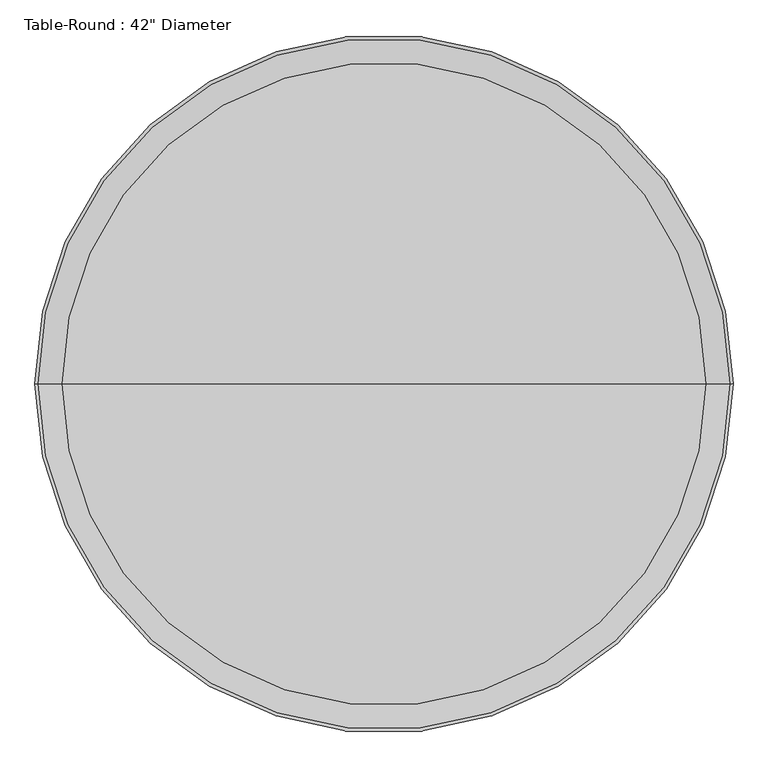
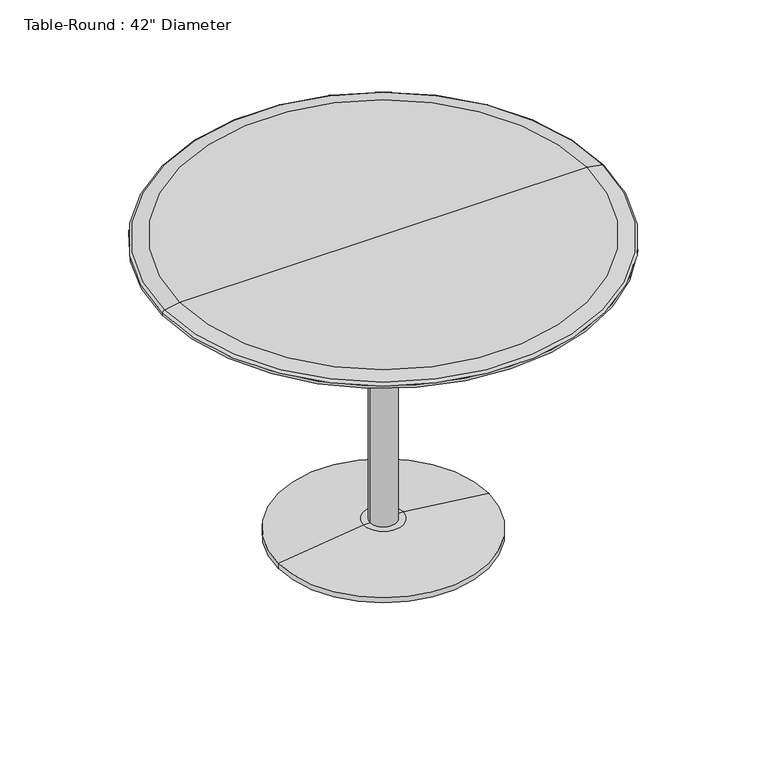
"""IFC4 building model written with IfcOpenShell, lengths in millimetres: furniture geometry."""

import ifcopenshell
import ifcopenshell.guid

model = None  # the IFC model being written
_history = None  # IfcOwnerHistory: only IFC2X3 demands one
_inside = {}  # id of a spatial element -> (the spatial element, [elements in it])
_under = {}  # id of a project, library or spatial element -> (it, [spatial elements below it])
_declared = {}  # id of a project -> (the project, [libraries it declares])
_typed = {}  # id of a type object -> (the type object, [elements of that type])
_made_of = {}  # id of a material, layer set ... -> (it, [elements and type objects made of it])


def new_model(schema):
    """Start an empty IFC model of exactly this schema.

    Asked for "IFC4X3", IfcOpenShell would pick the latest addendum, in which some entities
    have other attributes; the version numbers below select the first issue.
    IFC2X3 requires an IfcOwnerHistory on every rooted entity: one is made here for all.
    """
    global model, _history
    if schema == "IFC4X3":
        model = ifcopenshell.file(schema_version=(4, 3, 0, 0))
    else:
        model = ifcopenshell.file(schema=schema)
    _inside.clear()
    _under.clear()
    _declared.clear()
    _typed.clear()
    _made_of.clear()
    _history = None
    if model.schema == "IFC2X3":
        org = make("IfcOrganization", Name="unknown")
        user = make(
            "IfcPersonAndOrganization",
            ThePerson=make("IfcPerson", FamilyName="unknown"),
            TheOrganization=org,
        )
        app = make(
            "IfcApplication",
            ApplicationDeveloper=org,
            Version="unknown",
            ApplicationFullName="unknown",
            ApplicationIdentifier="unknown",
        )
        _history = make(
            "IfcOwnerHistory",
            OwningUser=user,
            OwningApplication=app,
            ChangeAction="ADDED",
            CreationDate=0,
        )
    return model


def make(cls, **values):
    """One entity of the class cls with the attributes given. An attribute that is None is left unset."""
    return model.create_entity(
        cls, **{name: value for name, value in values.items() if value is not None}
    )


def rooted(cls, **values):
    """An entity with a GlobalId (a new one), such as an element, a storey or a relation."""
    return make(cls, GlobalId=ifcopenshell.guid.new(), OwnerHistory=_history, **values)


def si_unit(unit_type, name, prefix=None):
    """IfcSIUnit, for example si_unit("LENGTHUNIT", "METRE", prefix="MILLI")."""
    return make("IfcSIUnit", UnitType=unit_type, Prefix=prefix, Name=name)


def assignment(units):
    """IfcUnitAssignment: the units of a project."""
    return None if units is None else make("IfcUnitAssignment", Units=units)


def point(xyz):
    """IfcCartesianPoint."""
    return None if xyz is None else make("IfcCartesianPoint", Coordinates=xyz)


def direction(xyz):
    """IfcDirection."""
    return None if xyz is None else make("IfcDirection", DirectionRatios=xyz)


def frame(location, z_axis=None, x_axis=None):
    """IfcAxis2Placement3D, a coordinate frame: its origin and axes. An axis left out is left unset."""
    return make(
        "IfcAxis2Placement3D",
        Location=point(location),
        Axis=direction(z_axis),
        RefDirection=direction(x_axis),
    )


def frame_2d(location, x_axis=None):
    """IfcAxis2Placement2D, a coordinate frame in the plane: its origin and x axis."""
    return make(
        "IfcAxis2Placement2D", Location=point(location), RefDirection=direction(x_axis)
    )


def origin():
    """The frame at (0, 0, 0) with its axes left unset."""
    return frame((0.0, 0.0, 0.0))


def origin_2d():
    """The frame at (0, 0) in the plane with its x axis left unset."""
    return frame_2d((0.0, 0.0))


def place(relative_to, where):
    """IfcLocalPlacement: puts the frame where relative to a parent placement (None: the world)."""
    return make(
        "IfcLocalPlacement", PlacementRelTo=relative_to, RelativePlacement=where
    )


def context(
    kind, dimensions, precision=None, world=None, true_north=None, identifier=None
):
    """IfcGeometricRepresentationContext, for example the 3D "Model" context."""
    return make(
        "IfcGeometricRepresentationContext",
        ContextIdentifier=identifier,
        ContextType=kind,
        CoordinateSpaceDimension=dimensions,
        Precision=precision,
        WorldCoordinateSystem=world,
        TrueNorth=true_north,
    )


def project(units=None, contexts=None):
    """IfcProject with its units and contexts."""
    return rooted(
        "IfcProject",
        Name="project",
        RepresentationContexts=contexts,
        UnitsInContext=assignment(units),
    )


def spatial(cls, under=None, at=None, **own):
    """A site, building, storey or space (cls), placed at a placement, below another one or the project."""
    s = rooted(cls, ObjectPlacement=at, **own)
    if under is not None:
        _under.setdefault(under.id(), (under, []))[1].append(s)
    return s


def polyline(points):
    """IfcPolyline through the points."""
    return make("IfcPolyline", Points=[point(p) for p in points])


def circle_curve(where, radius):
    """IfcCircle in the frame where."""
    return make("IfcCircle", Position=where, Radius=radius)


def ellipse_curve(where, semi_axis1, semi_axis2):
    """IfcEllipse in the frame where."""
    return make(
        "IfcEllipse", Position=where, SemiAxis1=semi_axis1, SemiAxis2=semi_axis2
    )


def trimmed(basis, trim1, trim2, sense, master):
    """IfcTrimmedCurve: the piece of a basis curve between two trims."""
    return make(
        "IfcTrimmedCurve",
        BasisCurve=basis,
        Trim1=trim1,
        Trim2=trim2,
        SenseAgreement=sense,
        MasterRepresentation=master,
    )


def segment(curve, same_sense, transition):
    """IfcCompositeCurveSegment."""
    return make(
        "IfcCompositeCurveSegment",
        Transition=transition,
        SameSense=same_sense,
        ParentCurve=curve,
    )


def composite_curve(segments, self_intersect=None):
    """IfcCompositeCurve: segments joined end to end."""
    return make("IfcCompositeCurve", Segments=segments, SelfIntersect=self_intersect)


def outline(outer, holes=None, kind="AREA"):
    """IfcArbitraryClosedProfileDef: a profile drawn as a closed curve; with holes, ...WithVoids."""
    if holes is None:
        return make("IfcArbitraryClosedProfileDef", ProfileType=kind, OuterCurve=outer)
    return make(
        "IfcArbitraryProfileDefWithVoids",
        ProfileType=kind,
        OuterCurve=outer,
        InnerCurves=holes,
    )


def extrude(swept, where, along, depth):
    """IfcExtrudedAreaSolid: the profile swept, set in the frame where, extruded along a direction by depth."""
    return make(
        "IfcExtrudedAreaSolid",
        SweptArea=swept,
        Position=where,
        ExtrudedDirection=direction(along),
        Depth=depth,
    )


def shape(context_of_items, identifier, shape_type, items):
    """IfcShapeRepresentation: the items that make up one representation, for example the "Body"."""
    return make(
        "IfcShapeRepresentation",
        ContextOfItems=context_of_items,
        RepresentationIdentifier=identifier,
        RepresentationType=shape_type,
        Items=items,
    )


def source(mapping_origin, context_of_items, identifier, shape_type, items):
    """IfcRepresentationMap: a shape defined once, which mapped items show again and again."""
    return make(
        "IfcRepresentationMap",
        MappingOrigin=mapping_origin,
        MappedRepresentation=shape(context_of_items, identifier, shape_type, items),
    )


def transform(
    local_origin,
    x_axis=None,
    y_axis=None,
    z_axis=None,
    scale=None,
    scale2=None,
    scale3=None,
    uniform=True,
):
    """IfcCartesianTransformationOperator3D, or its non-uniform kind. x_axis, y_axis, z_axis: its Axis1, 2, 3."""
    if uniform:
        return make(
            "IfcCartesianTransformationOperator3D",
            Axis1=direction(x_axis),
            Axis2=direction(y_axis),
            LocalOrigin=point(local_origin),
            Scale=scale,
            Axis3=direction(z_axis),
        )
    return make(
        "IfcCartesianTransformationOperator3DnonUniform",
        Axis1=direction(x_axis),
        Axis2=direction(y_axis),
        LocalOrigin=point(local_origin),
        Scale=scale,
        Axis3=direction(z_axis),
        Scale2=scale2,
        Scale3=scale3,
    )


def mapped(mapping_source, mapping_target):
    """IfcMappedItem: shows the shape of a source again, moved by a transform."""
    return make(
        "IfcMappedItem", MappingSource=mapping_source, MappingTarget=mapping_target
    )


def made_of(thing, what):
    """Note that an element or type object is made of a material, layer set ...; save() writes the relation."""
    if what is not None:
        _made_of.setdefault(what.id(), (what, []))[1].append(thing)
    return thing


def element(
    cls,
    number,
    at=None,
    inside=None,
    cuts=None,
    type_object=None,
    material=None,
    context=None,
    identifier="Body",
    shape_type=None,
    held_by="IfcProductDefinitionShape",
    body=None,
    shapes=None,
    **own,
):
    """One element of the class cls, such as IfcWall. Its Tag is "e" and its number.

    at: its placement. inside: the storey or other place that contains it. cuts: it is an
    opening in that element (IfcRelVoidsElement). A single representation is given by context,
    identifier, shape_type and body (its items); several are given by shapes. held_by: the class
    of the entity that holds the representations. save() writes the other relations.
    """
    e = rooted(cls, Tag="e%d" % number, ObjectPlacement=at, **own)
    if body is not None:
        shapes = [shape(context, identifier, shape_type, body)]
    if shapes is not None:
        e.Representation = make(held_by, Representations=shapes)
    if inside is not None:
        _inside.setdefault(inside.id(), (inside, []))[1].append(e)
    if cuts is not None:
        rooted(
            "IfcRelVoidsElement", RelatingBuildingElement=cuts, RelatedOpeningElement=e
        )
    if type_object is not None:
        _typed.setdefault(type_object.id(), (type_object, []))[1].append(e)
    return made_of(e, material)


def aggregate(whole, parts):
    """IfcRelAggregates: a whole, such as a stair, and the parts it consists of."""
    return rooted("IfcRelAggregates", RelatingObject=whole, RelatedObjects=parts)


def save(model, path):
    """Write the relations noted so far, then the file.

    IfcRelAggregates (storeys below a building ...), IfcRelContainedInSpatialStructure (elements
    in a storey), IfcRelDefinesByType, IfcRelAssociatesMaterial and IfcRelDeclares: one each for
    every whole, place, type object, material and project.
    """
    for whole, parts in _under.values():
        aggregate(whole, parts)
    for where, things in _inside.values():
        rooted(
            "IfcRelContainedInSpatialStructure",
            RelatedElements=things,
            RelatingStructure=where,
        )
    for kind, things in _typed.values():
        rooted("IfcRelDefinesByType", RelatedObjects=things, RelatingType=kind)
    for what, things in _made_of.values():
        rooted("IfcRelAssociatesMaterial", RelatedObjects=things, RelatingMaterial=what)
    for by, libraries in _declared.values():
        rooted("IfcRelDeclares", RelatingContext=by, RelatedDefinitions=libraries)
    model.write(path)


def plane_surface(at):
    """IfcPlane: the flat surface through the origin of the frame at, square to its z axis."""
    return make("IfcPlane", Position=at)


def cylinder_surface(at, radius):
    """IfcCylindricalSurface: all points at the distance radius from the z axis of the frame at."""
    return make("IfcCylindricalSurface", Position=at, Radius=radius)


def revolved_surface(curve, axis_point, axis_direction):
    """IfcSurfaceOfRevolution: the curve turned about the line through axis_point along axis_direction."""
    return make(
        "IfcSurfaceOfRevolution",
        SweptCurve=make("IfcArbitraryOpenProfileDef", ProfileType="CURVE", Curve=curve),
        AxisPosition=make("IfcAxis1Placement", Location=point(axis_point), Axis=direction(axis_direction)),
    )


def advanced_brep(points, edges, surfaces, faces):
    """IfcAdvancedBrep: a solid bounded by faces that lie on surfaces and meet in shared edges.

    An edge is (start, end): straight between two places in points (the first is 0);
    or (start, end, curve); or (start, end, curve, False) where it runs against its curve.
    A face is (place in surfaces, loops), or (place, loops, False) where it looks against
    its surface's normal. A loop lists edges by number (the first is 1), with a minus sign
    where the edge is run from its end to its start. The first loop is the outer one.
    """
    corners = [point(p) for p in points]
    vertices = [make("IfcVertexPoint", VertexGeometry=c) for c in corners]
    made = []
    for start, end, *more in edges:
        made.append(
            make(
                "IfcEdgeCurve",
                EdgeStart=vertices[start],
                EdgeEnd=vertices[end],
                EdgeGeometry=more[0] if more else make("IfcPolyline", Points=[corners[start], corners[end]]),
                SameSense=more[1] if len(more) > 1 else True,
            )
        )
    hull = []
    for where, loops, *sense in faces:
        bounds = []
        for j, loop in enumerate(loops):
            ring = [make("IfcOrientedEdge", EdgeElement=made[abs(k) - 1], Orientation=k > 0) for k in loop]
            bounds.append(
                make(
                    "IfcFaceOuterBound" if j == 0 else "IfcFaceBound",
                    Bound=make("IfcEdgeLoop", EdgeList=ring),
                    Orientation=True,
                )
            )
        hull.append(make("IfcAdvancedFace", Bounds=bounds, FaceSurface=surfaces[where], SameSense=sense[0] if sense else True))
    return make("IfcAdvancedBrep", Outer=make("IfcClosedShell", CfsFaces=hull))


def furniture_77f0a01d(model_context):
    return source(origin(), model_context, "Body", "SolidModel", [
        extrude(outline(composite_curve([segment(trimmed(circle_curve(origin_2d(), 31.75), [point((-31.75, 0.0))], [point((31.75, 0.0))], False, "CARTESIAN"), True, "CONTINUOUS"), segment(trimmed(circle_curve(origin_2d(), 31.75), [point((31.75, 0.0))], [point((-31.75, 0.0))], False, "CARTESIAN"), True, "CONTINUOUS")], self_intersect=False)), frame((0.0, 0.0, 38.1), z_axis=(0.0, 0.0, 1.0), x_axis=(1.0, 0.0, 0.0)), (0.0, 0.0, 1.0), 704.85),
        advanced_brep(
        [(0.0, 0.0, 742.95), (-533.4, 0.0, 742.95), (533.4, 0.0, 742.95), (491.5011364, 0.0, 762.0), (-491.5011364, 0.0, 762.0), (0.0, 0.0, 762.0), (528.1526659, 0.0, 755.5373465), (-528.1526659, 0.0, 755.5373465), (533.4, 0.0, 749.2838172), (-533.4, 0.0, 749.2838172)],
        [
            (0, 1),
            (1, 2, circle_curve(frame((0.0, 0.0, 742.95), z_axis=(0.0, 0.0, -1.0), x_axis=(-1.0, 0.0, 0.0)), 533.4)),
            (2, 0),
            (2, 1, circle_curve(frame((0.0, 0.0, 742.95), z_axis=(0.0, 0.0, -1.0), x_axis=(-1.0, 0.0, 0.0)), 533.4)),
            (3, 4, circle_curve(frame((0.0, 0.0, 762.0), z_axis=(0.0, 0.0, 1.0), x_axis=(-1.0, 0.0, 0.0)), 491.5011364)),
            (4, 5),
            (5, 3),
            (4, 3, circle_curve(frame((0.0, 0.0, 762.0), z_axis=(0.0, 0.0, 1.0), x_axis=(-1.0, 0.0, 0.0)), 491.5011364)),
            (6, 7, circle_curve(frame((0.0, 0.0, 755.5373465), z_axis=(0.0, 0.0, 1.0), x_axis=(-1.0, 0.0, 0.0)), 528.1526659)),
            (7, 4),
            (3, 6),
            (7, 6, circle_curve(frame((0.0, 0.0, 755.5373465), z_axis=(0.0, 0.0, 1.0), x_axis=(-1.0, 0.0, 0.0)), 528.1526659)),
            (8, 9, circle_curve(frame((0.0, 0.0, 749.2838172), z_axis=(0.0, 0.0, 1.0), x_axis=(-1.0, 0.0, 0.0)), 533.4)),
            (9, 7, circle_curve(frame((-527.05, 0.0, 749.2838172), z_axis=(0.0, 1.0, 0.0), x_axis=(1.0, 0.0, 0.0)), 6.35)),
            (6, 8, circle_curve(frame((527.05, 0.0, 749.2838172), z_axis=(0.0, 1.0, 0.0), x_axis=(-1.0, 0.0, 0.0)), 6.35)),
            (9, 8, circle_curve(frame((0.0, 0.0, 749.2838172), z_axis=(0.0, 0.0, 1.0), x_axis=(-1.0, 0.0, 0.0)), 533.4)),
            (1, 9),
            (8, 2),
        ],
        [
            plane_surface(frame((0.0, 0.0, 742.95), z_axis=(0.0, 0.0, -1.0), x_axis=(-1.0, 0.0, 0.0))),
            plane_surface(frame((0.0, 0.0, 762.0), z_axis=(0.0, 0.0, 1.0), x_axis=(-1.0, 0.0, 0.0))),
            revolved_surface(polyline([(-491.5011364, 0.0, 762.0), (-528.1526659, 0.0, 755.5373465)]), (0.0, 0.0, 838.2), (0.0, 0.0, -1.0)),
            revolved_surface(trimmed(ellipse_curve(frame((-527.05, 0.0, 749.2838172), z_axis=(0.0, -1.0, 0.0), x_axis=(1.0, 0.0, 0.0)), 6.35, 6.35), [point((-528.1526659, 0.0, 755.5373465))], [point((-533.4, 0.0, 749.2838172))], True, "CARTESIAN"), (0.0, 0.0, 838.2), (0.0, 0.0, -1.0)),
            cylinder_surface(frame((0.0, 0.0, 838.2), z_axis=(0.0, 0.0, -1.0), x_axis=(-1.0, 0.0, 0.0)), 533.4),
        ],
        [
            (0, [[1, 2, 3]]),
            (0, [[-3, 4, -1]]),
            (1, [[5, 6, 7]]),
            (1, [[8, -7, -6]]),
            (2, [[9, 10, -5, 11]]),
            (2, [[12, -11, -8, -10]]),
            (3, [[13, 14, -9, 15]]),
            (3, [[16, -15, -12, -14]]),
            (4, [[-2, 17, -13, 18]]),
            (4, [[-4, -18, -16, -17]]),
        ],
    ),
        advanced_brep(
        [(0.0, 0.0, 0.0), (-254.0, 0.0, 0.0), (254.0, 0.0, 0.0), (47.625, 0.0, 38.1), (-47.625, 0.0, 38.1), (0.0, 0.0, 38.1), (254.0, 0.0, 12.7), (-254.0, 0.0, 12.7)],
        [
            (0, 1),
            (1, 2, circle_curve(frame((0.0, 0.0, 0.0), z_axis=(0.0, 0.0, -1.0), x_axis=(-1.0, 0.0, 0.0)), 254.0)),
            (2, 0),
            (2, 1, circle_curve(frame((0.0, 0.0, 0.0), z_axis=(0.0, 0.0, -1.0), x_axis=(-1.0, 0.0, 0.0)), 254.0)),
            (3, 4, circle_curve(frame((0.0, 0.0, 38.1), z_axis=(0.0, 0.0, 1.0), x_axis=(-1.0, 0.0, 0.0)), 47.625)),
            (4, 5),
            (5, 3),
            (4, 3, circle_curve(frame((0.0, 0.0, 38.1), z_axis=(0.0, 0.0, 1.0), x_axis=(-1.0, 0.0, 0.0)), 47.625)),
            (6, 7, circle_curve(frame((0.0, 0.0, 12.7), z_axis=(0.0, 0.0, 1.0), x_axis=(-1.0, 0.0, 0.0)), 254.0)),
            (7, 4),
            (3, 6),
            (7, 6, circle_curve(frame((0.0, 0.0, 12.7), z_axis=(0.0, 0.0, 1.0), x_axis=(-1.0, 0.0, 0.0)), 254.0)),
            (1, 7),
            (6, 2),
        ],
        [
            plane_surface(frame((0.0, 0.0, 0.0), z_axis=(0.0, 0.0, -1.0), x_axis=(-1.0, 0.0, 0.0))),
            plane_surface(frame((0.0, 0.0, 38.1), z_axis=(0.0, 0.0, 1.0), x_axis=(-1.0, 0.0, 0.0))),
            revolved_surface(polyline([(-47.625, 0.0, 38.1), (-254.0, 0.0, 12.7)]), (0.0, 0.0, 215.9), (0.0, 0.0, -1.0)),
            cylinder_surface(frame((0.0, 0.0, 215.9), z_axis=(0.0, 0.0, -1.0), x_axis=(-1.0, 0.0, 0.0)), 254.0),
        ],
        [
            (0, [[1, 2, 3]]),
            (0, [[-3, 4, -1]]),
            (1, [[5, 6, 7]]),
            (1, [[8, -7, -6]]),
            (2, [[9, 10, -5, 11]]),
            (2, [[12, -11, -8, -10]]),
            (3, [[-2, 13, -9, 14]]),
            (3, [[-4, -14, -12, -13]]),
        ],
    ),
    ])


if __name__ == "__main__":
    model = new_model("IFC4")
    model_context = context("Model", 3, world=origin())
    ifc_project = project(units=[si_unit("LENGTHUNIT", "METRE", prefix="MILLI")], contexts=[model_context])
    site = spatial("IfcSite", under=ifc_project)
    building = spatial("IfcBuilding", under=site)
    placement = place(None, origin())
    furniture_shape = furniture_77f0a01d(model_context)
    element("IfcFurniture", 1, ObjectType="Table-Round : 42\" Diameter", at=placement, inside=building, context=model_context, shape_type="MappedRepresentation", body=[
        mapped(furniture_shape, transform((0.0, 0.0, 0.0), x_axis=(1.0, 0.0, 0.0), y_axis=(0.0, 1.0, 0.0), z_axis=(0.0, 0.0, 1.0))),
    ])
    save(model, "model.ifc")

# Revit data of these elements
# Type "Table-Round : 42\" Diameter"
#   Assembly Code = "E2020200"
#   Base Radius = 0' - 10"
#   Height = 2' - 6"
#   Radius = 1' - 9"
#   Base Material = Steel, Chrome Plated
#   Top Material = Birch
#   Default Elevation = 0
# Element 1 (IfcFurniture, "Table-Round : 42\" Diameter")
#   Materials on its faces: "Steel, Chrome Plated", "Birch"
# Materials
#   "Steel, Chrome Plated": class "Metal", colour RGB 17 17 17, transparency 0, Description = "Chromiuim plated steel", Cost = 0
#   "Birch": class "Wood", colour RGB 224 178 126, transparency 0, Description = "Betula Alleghaniensis", Cost = 0
